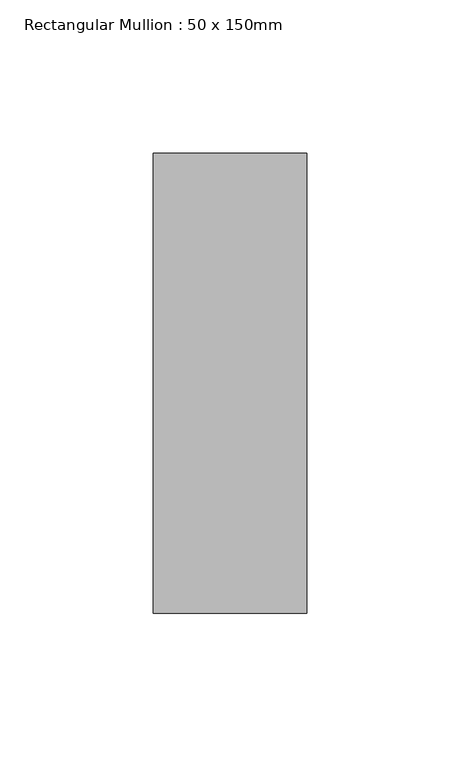
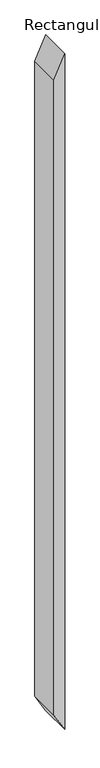
"""IFC4 building model written with IfcOpenShell, lengths in millimetres: member geometry, Rectangular Mullion : 50 x 150mm."""

from ifc_helpers import new_model, si_unit, frame, origin, place, context, project, spatial, polyline, outline, extrude, source, transform, mapped, element, save


def rectangular_mullion_50_x_150mm_45cfd48e(model_context):
    return source(origin(), model_context, "Body", "SweptSolid", [
        extrude(outline(polyline([(0.0, 0.0), (-108.6604448, -50.0), (-3159.4549255, -50.0), (-3244.7760444, 0.0), (0.0, 0.0)])), frame((0.0, -75.0, 0.0), z_axis=(0.0, 1.0, 0.0), x_axis=(0.0, 0.0, 1.0)), (0.0, 0.0, 1.0), 150.0),
    ])


if __name__ == "__main__":
    model = new_model("IFC4")
    model_context = context("Model", 3, world=origin())
    ifc_project = project(units=[si_unit("LENGTHUNIT", "METRE", prefix="MILLI")], contexts=[model_context])
    site = spatial("IfcSite", under=ifc_project)
    building = spatial("IfcBuilding", under=site)
    placement = place(None, origin())
    rectangular_mullion_50_x_150mm_shape = rectangular_mullion_50_x_150mm_45cfd48e(model_context)
    element("IfcMember", 1, ObjectType="Rectangular Mullion : 50 x 150mm", at=placement, inside=building, context=model_context, shape_type="MappedRepresentation", body=[
        mapped(rectangular_mullion_50_x_150mm_shape, transform((0.0, 0.0, 0.0), x_axis=(1.0, 0.0, 0.0), y_axis=(0.0, 1.0, 0.0), z_axis=(0.0, 0.0, 1.0))),
    ])
    save(model, "model.ifc")

# Revit data of these elements
# Type "Rectangular Mullion : 50 x 150mm"
#   built-in parameter 1007304 = 0.492126 (stored number, unit not read)
#   built-in parameter 1007301 = 0.082021 (stored number, unit not read)
#   built-in parameter 1007300 = 0.082021 (stored number, unit not read)
# Element 1 (IfcMember, "Rectangular Mullion : 50 x 150mm")
#   Materials on its faces: "Metal - Aluminium"
# Materials
#   "Metal - Aluminium": class "Metal", colour RGB 247 247 247, transparency 0
